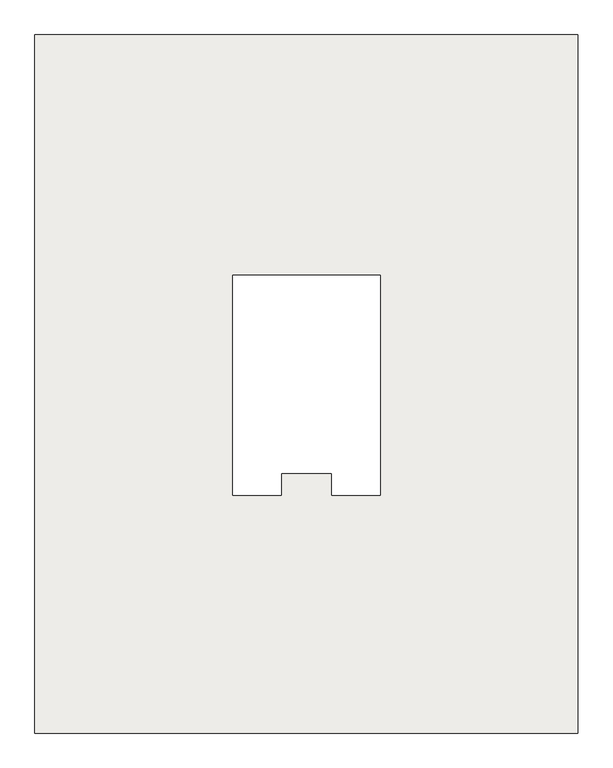
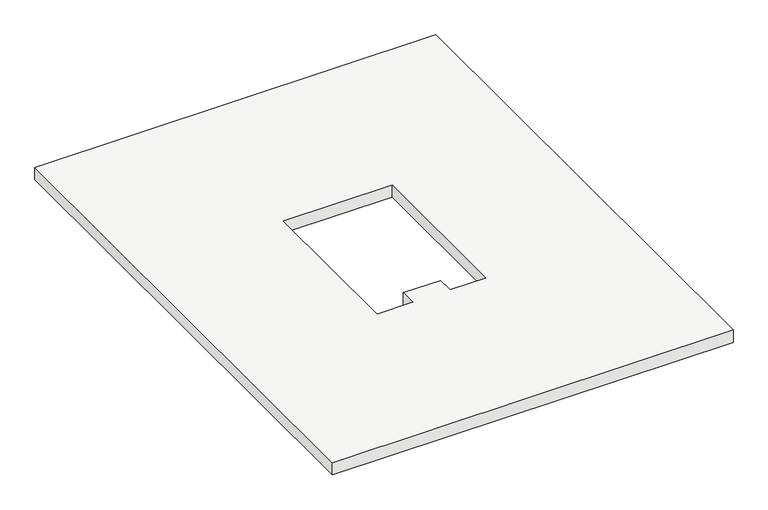
"""IFC4 building model written with IfcOpenShell, lengths in millimetres: slab geometry, Holzdecke."""

from ifc_helpers import new_model, si_unit, origin, origin_with_axes, place, context, project, spatial, polyline, outline, extrude, source, transform, mapped, element, save


def slab_cbd63e04(model_context):
    return source(origin(), model_context, "Body", "SweptSolid", [
        extrude(outline(polyline([(0.0, 18002.8619019), (14000.0, 18002.8619019), (14000.0, 0.0), (0.0, 0.0), (0.0, 18002.8619019)]), holes=[polyline([(8900.0, 11802.8619019), (5100.0, 11802.8619019), (5100.0, 6132.8619019), (6350.0, 6132.8619019), (6350.0, 6703.1288328), (7650.0, 6703.1288328), (7650.0, 6132.8619019), (8900.0, 6132.8619019), (8900.0, 11802.8619019)])]), origin_with_axes(), (0.0, 0.0, 1.0), 450.0),
    ])


if __name__ == "__main__":
    model = new_model("IFC4")
    model_context = context("Model", 3, world=origin())
    ifc_project = project(units=[si_unit("LENGTHUNIT", "METRE", prefix="MILLI")], contexts=[model_context])
    site = spatial("IfcSite", under=ifc_project)
    building = spatial("IfcBuilding", under=site)
    placement = place(None, origin())
    slab_shape = slab_cbd63e04(model_context)
    element("IfcSlab", 1, ObjectType="Holzdecke", at=placement, inside=building, context=model_context, shape_type="MappedRepresentation", body=[
        mapped(slab_shape, transform((0.0, 0.0, 0.0), x_axis=(1.0, 0.0, 0.0), y_axis=(0.0, 1.0, 0.0), z_axis=(0.0, 0.0, 1.0))),
    ])
    save(model, "model.ifc")

# Revit data of these elements
# Element 1 (IfcSlab, "Holzdecke")
#   Materials on its faces: "holzschalung"
# Materials
#   "holzschalung": class "Unassigned", colour RGB 128 128 128, transparency 0
